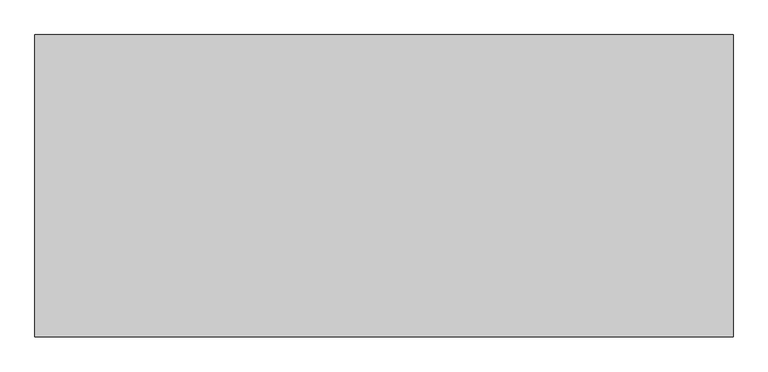
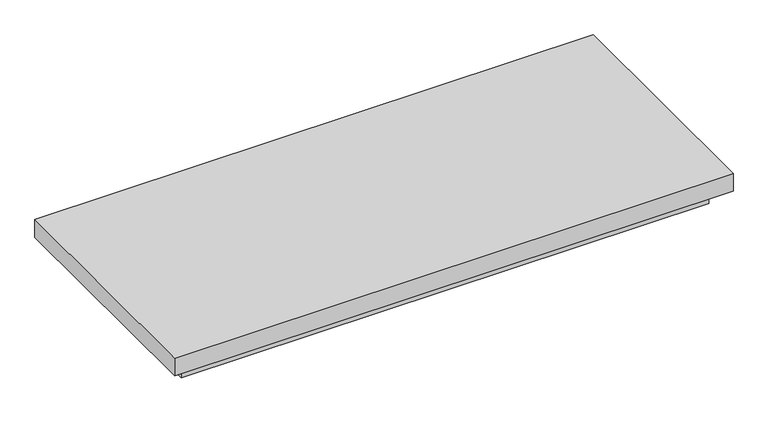
"""IFC4 building model written with IfcOpenShell, lengths in millimetres: proxy geometry, TAMPO - CASA DE MÁQUINA : TAMPO - CASA DE MÁQUINA."""

from ifc_helpers import new_model, si_unit, frame, origin, place, context, project, spatial, polyline, outline, extrude, source, transform, mapped, element, save


def specialty_equipment_67e2e29c(model_context):
    return source(origin(), model_context, "Body", "SweptSolid", [
        extrude(outline(polyline([(12687.718693, 5627.4300153), (12687.718693, 4481.4300153), (10041.718693, 4481.4300153), (10041.718693, 5627.4300153), (12687.718693, 5627.4300153)])), frame((0.0, 0.0, 280.0), z_axis=(0.0, 0.0, 1.0), x_axis=(1.0, 0.0, 0.0)), (0.0, 0.0, 1.0), 88.4706632),
        extrude(outline(polyline([(12614.718693, 5554.4300153), (12614.718693, 4554.4300153), (10114.718693, 4554.4300153), (10114.718693, 5554.4300153), (12614.718693, 5554.4300153)])), frame((0.0, 0.0, 200.0), z_axis=(0.0, 0.0, 1.0), x_axis=(1.0, 0.0, 0.0)), (0.0, 0.0, 1.0), 80.0),
    ])


if __name__ == "__main__":
    model = new_model("IFC4")
    model_context = context("Model", 3, world=origin())
    ifc_project = project(units=[si_unit("LENGTHUNIT", "METRE", prefix="MILLI")], contexts=[model_context])
    site = spatial("IfcSite", under=ifc_project)
    building = spatial("IfcBuilding", under=site)
    placement = place(None, origin())
    specialty_equipment_shape = specialty_equipment_67e2e29c(model_context)
    element("IfcBuildingElementProxy", 1, Name="TAMPO - CASA DE MÁQUINA : TAMPO - CASA DE MÁQUINA", ObjectType="TAMPO - CASA DE MÁQUINA : TAMPO - CASA DE MÁQUINA", at=placement, inside=building, context=model_context, shape_type="MappedRepresentation", body=[
        mapped(specialty_equipment_shape, transform((0.0, 0.0, 0.0), x_axis=(1.0, 0.0, 0.0), y_axis=(0.0, 1.0, 0.0), z_axis=(0.0, 0.0, 1.0))),
    ])
    save(model, "model.ifc")

# Revit data of these elements
# Element 1 (IfcBuildingElementProxy, "TAMPO - CASA DE MÁQUINA : TAMPO - CASA DE MÁQUINA")
#   Materials on its faces: ".ALUMÍNIO"
# Materials
#   ".ALUMÍNIO": class "CC_METAIS", colour RGB 244 244 244, transparency 0, Description = "Material alumínio", Cost = 0
